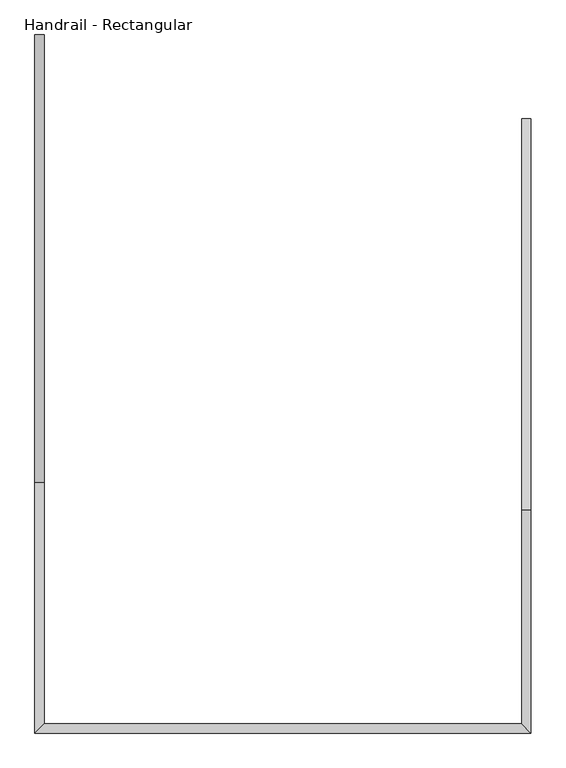
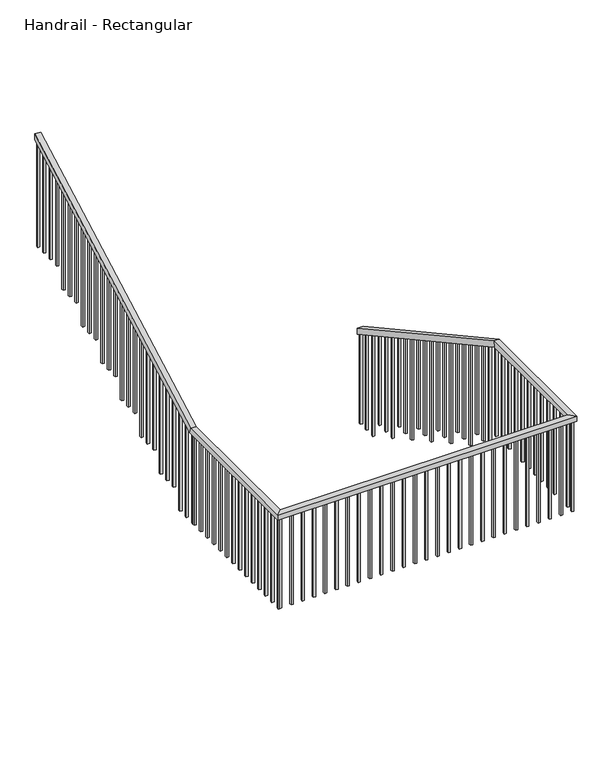
"""IFC4 building model written with IfcOpenShell, lengths in millimetres: railing geometry, Handrail - Rectangular."""

from ifc_helpers import new_model, si_unit, frame, origin, place, context, project, spatial, polyline, outline, extrude, faceted_brep, source, transform, mapped, element, save


def handrail_rectangular_cd72d91a(model_context):
    return source(origin(), model_context, "Body", "SolidModel", [
        faceted_brep([(-73285.35, 12185.65, 17490.1411765), (-73285.35, 12185.65, 17432.1885835), (-73336.15, 12185.65, 17432.1885835), (-73336.15, 12185.65, 17490.1411765), (-73285.35, 10052.05, 18661.5294118), (-73285.35, 10039.0220627, 18610.7294118), (-73336.15, 10039.0220627, 18610.7294118), (-73336.15, 10052.05, 18661.5294118), (-73285.35, 8839.2, 18661.5294118), (-73285.35, 8839.2, 18610.7294118), (-73336.15, 8890.0, 18610.7294118), (-73336.15, 8890.0, 18661.5294118), (-75990.45, 8839.2, 18661.5294118), (-75990.45, 8839.2, 18610.7294118), (-75939.65, 8890.0, 18610.7294118), (-75939.65, 8890.0, 18661.5294118), (-75990.45, 10204.45, 18661.5294118), (-75990.45, 10217.4779373, 18610.7294118), (-75939.65, 10217.4779373, 18610.7294118), (-75939.65, 10204.45, 18661.5294118), (-75990.45, 12642.85, 20000.2588235), (-75939.65, 12642.85, 20000.2588235), (-75939.65, 12642.85, 19942.3062305), (-75990.45, 12642.85, 19942.3062305)], [[[0, 1, 2, 3]], [[1, 0, 4, 5]], [[2, 1, 5, 6]], [[3, 2, 6, 7]], [[0, 3, 7, 4]], [[5, 4, 8, 9]], [[6, 5, 9, 10]], [[7, 6, 10, 11]], [[4, 7, 11, 8]], [[9, 8, 12, 13]], [[10, 9, 13, 14]], [[11, 10, 14, 15]], [[8, 11, 15, 12]], [[13, 12, 16, 17]], [[14, 13, 17, 18]], [[15, 14, 18, 19]], [[12, 15, 19, 16]], [[20, 21, 22, 23]], [[17, 16, 20, 23]], [[18, 17, 23, 22]], [[19, 18, 22, 21]], [[16, 19, 21, 20]]]),
        extrude(outline(polyline([(12550.775, 19891.7552501), (12550.775, 18918.5176471), (12531.725, 18918.5176471), (12531.725, 19881.2964266), (12550.775, 19891.7552501)])), frame((-75974.575, 0.0, 0.0), z_axis=(1.0, 0.0, 0.0), x_axis=(0.0, 1.0, 0.0)), (0.0, 0.0, 1.0), 19.05),
        extrude(outline(polyline([(12449.175, 19835.974858), (12449.175, 18918.5176471), (12430.125, 18918.5176471), (12430.125, 19825.5160344), (12449.175, 19835.974858)])), frame((-75974.575, 0.0, 0.0), z_axis=(1.0, 0.0, 0.0), x_axis=(0.0, 1.0, 0.0)), (0.0, 0.0, 1.0), 19.05),
        extrude(outline(polyline([(12347.575, 19780.1944658), (12347.575, 18918.5176471), (12328.525, 18918.5176471), (12328.525, 19769.7356423), (12347.575, 19780.1944658)])), frame((-75974.575, 0.0, 0.0), z_axis=(1.0, 0.0, 0.0), x_axis=(0.0, 1.0, 0.0)), (0.0, 0.0, 1.0), 19.05),
        extrude(outline(polyline([(12245.975, 19724.4140737), (12245.975, 18751.1764706), (12226.925, 18751.1764706), (12226.925, 19713.9552501), (12245.975, 19724.4140737)])), frame((-75974.575, 0.0, 0.0), z_axis=(1.0, 0.0, 0.0), x_axis=(0.0, 1.0, 0.0)), (0.0, 0.0, 1.0), 19.05),
        extrude(outline(polyline([(12144.375, 19668.6336815), (12144.375, 18751.1764706), (12125.325, 18751.1764706), (12125.325, 19658.174858), (12144.375, 19668.6336815)])), frame((-75974.575, 0.0, 0.0), z_axis=(1.0, 0.0, 0.0), x_axis=(0.0, 1.0, 0.0)), (0.0, 0.0, 1.0), 19.05),
        extrude(outline(polyline([(12042.775, 19612.8532893), (12042.775, 18751.1764706), (12023.725, 18751.1764706), (12023.725, 19602.3944658), (12042.775, 19612.8532893)])), frame((-75974.575, 0.0, 0.0), z_axis=(1.0, 0.0, 0.0), x_axis=(0.0, 1.0, 0.0)), (0.0, 0.0, 1.0), 19.05),
        extrude(outline(polyline([(11941.175, 19557.0728972), (11941.175, 18583.8352941), (11922.125, 18583.8352941), (11922.125, 19546.6140737), (11941.175, 19557.0728972)])), frame((-75974.575, 0.0, 0.0), z_axis=(1.0, 0.0, 0.0), x_axis=(0.0, 1.0, 0.0)), (0.0, 0.0, 1.0), 19.05),
        extrude(outline(polyline([(11839.575, 19501.292505), (11839.575, 18583.8352941), (11820.525, 18583.8352941), (11820.525, 19490.8336815), (11839.575, 19501.292505)])), frame((-75974.575, 0.0, 0.0), z_axis=(1.0, 0.0, 0.0), x_axis=(0.0, 1.0, 0.0)), (0.0, 0.0, 1.0), 19.05),
        extrude(outline(polyline([(11737.975, 19445.5121129), (11737.975, 18583.8352941), (11718.925, 18583.8352941), (11718.925, 19435.0532893), (11737.975, 19445.5121129)])), frame((-75974.575, 0.0, 0.0), z_axis=(1.0, 0.0, 0.0), x_axis=(0.0, 1.0, 0.0)), (0.0, 0.0, 1.0), 19.05),
        extrude(outline(polyline([(11636.375, 19389.7317207), (11636.375, 18416.4941176), (11617.325, 18416.4941176), (11617.325, 19379.2728972), (11636.375, 19389.7317207)])), frame((-75974.575, 0.0, 0.0), z_axis=(1.0, 0.0, 0.0), x_axis=(0.0, 1.0, 0.0)), (0.0, 0.0, 1.0), 19.05),
        extrude(outline(polyline([(11534.775, 19333.9513286), (11534.775, 18416.4941176), (11515.725, 18416.4941176), (11515.725, 19323.492505), (11534.775, 19333.9513286)])), frame((-75974.575, 0.0, 0.0), z_axis=(1.0, 0.0, 0.0), x_axis=(0.0, 1.0, 0.0)), (0.0, 0.0, 1.0), 19.05),
        extrude(outline(polyline([(11433.175, 19278.1709364), (11433.175, 18416.4941176), (11414.125, 18416.4941176), (11414.125, 19267.7121129), (11433.175, 19278.1709364)])), frame((-75974.575, 0.0, 0.0), z_axis=(1.0, 0.0, 0.0), x_axis=(0.0, 1.0, 0.0)), (0.0, 0.0, 1.0), 19.05),
        extrude(outline(polyline([(11331.575, 19222.3905442), (11331.575, 18249.1529412), (11312.525, 18249.1529412), (11312.525, 19211.9317207), (11331.575, 19222.3905442)])), frame((-75974.575, 0.0, 0.0), z_axis=(1.0, 0.0, 0.0), x_axis=(0.0, 1.0, 0.0)), (0.0, 0.0, 1.0), 19.05),
        extrude(outline(polyline([(11229.975, 19166.6101521), (11229.975, 18249.1529412), (11210.925, 18249.1529412), (11210.925, 19156.1513286), (11229.975, 19166.6101521)])), frame((-75974.575, 0.0, 0.0), z_axis=(1.0, 0.0, 0.0), x_axis=(0.0, 1.0, 0.0)), (0.0, 0.0, 1.0), 19.05),
        extrude(outline(polyline([(11128.375, 19110.8297599), (11128.375, 18249.1529412), (11109.325, 18249.1529412), (11109.325, 19100.3709364), (11128.375, 19110.8297599)])), frame((-75974.575, 0.0, 0.0), z_axis=(1.0, 0.0, 0.0), x_axis=(0.0, 1.0, 0.0)), (0.0, 0.0, 1.0), 19.05),
        extrude(outline(polyline([(11026.775, 19055.0493678), (11026.775, 18081.8117647), (11007.725, 18081.8117647), (11007.725, 19044.5905442), (11026.775, 19055.0493678)])), frame((-75974.575, 0.0, 0.0), z_axis=(1.0, 0.0, 0.0), x_axis=(0.0, 1.0, 0.0)), (0.0, 0.0, 1.0), 19.05),
        extrude(outline(polyline([(10925.175, 18999.2689756), (10925.175, 18081.8117647), (10906.125, 18081.8117647), (10906.125, 18988.8101521), (10925.175, 18999.2689756)])), frame((-75974.575, 0.0, 0.0), z_axis=(1.0, 0.0, 0.0), x_axis=(0.0, 1.0, 0.0)), (0.0, 0.0, 1.0), 19.05),
        extrude(outline(polyline([(10823.575, 18943.4885835), (10823.575, 18081.8117647), (10804.525, 18081.8117647), (10804.525, 18933.0297599), (10823.575, 18943.4885835)])), frame((-75974.575, 0.0, 0.0), z_axis=(1.0, 0.0, 0.0), x_axis=(0.0, 1.0, 0.0)), (0.0, 0.0, 1.0), 19.05),
        extrude(outline(polyline([(10721.975, 18887.7081913), (10721.975, 17914.4705882), (10702.925, 17914.4705882), (10702.925, 18877.2493678), (10721.975, 18887.7081913)])), frame((-75974.575, 0.0, 0.0), z_axis=(1.0, 0.0, 0.0), x_axis=(0.0, 1.0, 0.0)), (0.0, 0.0, 1.0), 19.05),
        extrude(outline(polyline([(10620.375, 18831.9277991), (10620.375, 17914.4705882), (10601.325, 17914.4705882), (10601.325, 18821.4689756), (10620.375, 18831.9277991)])), frame((-75974.575, 0.0, 0.0), z_axis=(1.0, 0.0, 0.0), x_axis=(0.0, 1.0, 0.0)), (0.0, 0.0, 1.0), 19.05),
        extrude(outline(polyline([(10518.775, 18776.147407), (10518.775, 17914.4705882), (10499.725, 17914.4705882), (10499.725, 18765.6885835), (10518.775, 18776.147407)])), frame((-75974.575, 0.0, 0.0), z_axis=(1.0, 0.0, 0.0), x_axis=(0.0, 1.0, 0.0)), (0.0, 0.0, 1.0), 19.05),
        extrude(outline(polyline([(10417.175, 18720.3670148), (10417.175, 17747.1294118), (10398.125, 17747.1294118), (10398.125, 18709.9081913), (10417.175, 18720.3670148)])), frame((-75974.575, 0.0, 0.0), z_axis=(1.0, 0.0, 0.0), x_axis=(0.0, 1.0, 0.0)), (0.0, 0.0, 1.0), 19.05),
        extrude(outline(polyline([(10315.575, 18664.5866227), (10315.575, 17747.1294118), (10296.525, 17747.1294118), (10296.525, 18654.1277991), (10315.575, 18664.5866227)])), frame((-75974.575, 0.0, 0.0), z_axis=(1.0, 0.0, 0.0), x_axis=(0.0, 1.0, 0.0)), (0.0, 0.0, 1.0), 19.05),
        extrude(outline(polyline([(-75974.575, 10175.875), (-75974.575, 10194.925), (-75955.525, 10194.925), (-75955.525, 10175.875), (-75974.575, 10175.875)])), frame((0.0, 0.0, 17747.1294118), z_axis=(0.0, 0.0, 1.0), x_axis=(1.0, 0.0, 0.0)), (0.0, 0.0, 1.0), 863.6),
        extrude(outline(polyline([(-75974.575, 10074.275), (-75974.575, 10093.325), (-75955.525, 10093.325), (-75955.525, 10074.275), (-75974.575, 10074.275)])), frame((0.0, 0.0, 17747.1294118), z_axis=(0.0, 0.0, 1.0), x_axis=(1.0, 0.0, 0.0)), (0.0, 0.0, 1.0), 863.6),
        extrude(outline(polyline([(-75974.575, 9972.675), (-75974.575, 9991.725), (-75955.525, 9991.725), (-75955.525, 9972.675), (-75974.575, 9972.675)])), frame((0.0, 0.0, 17747.1294118), z_axis=(0.0, 0.0, 1.0), x_axis=(1.0, 0.0, 0.0)), (0.0, 0.0, 1.0), 863.6),
        extrude(outline(polyline([(-75974.575, 9871.075), (-75974.575, 9890.125), (-75955.525, 9890.125), (-75955.525, 9871.075), (-75974.575, 9871.075)])), frame((0.0, 0.0, 17747.1294118), z_axis=(0.0, 0.0, 1.0), x_axis=(1.0, 0.0, 0.0)), (0.0, 0.0, 1.0), 863.6),
        extrude(outline(polyline([(-75974.575, 9769.475), (-75974.575, 9788.525), (-75955.525, 9788.525), (-75955.525, 9769.475), (-75974.575, 9769.475)])), frame((0.0, 0.0, 17747.1294118), z_axis=(0.0, 0.0, 1.0), x_axis=(1.0, 0.0, 0.0)), (0.0, 0.0, 1.0), 863.6),
        extrude(outline(polyline([(-75974.575, 9667.875), (-75974.575, 9686.925), (-75955.525, 9686.925), (-75955.525, 9667.875), (-75974.575, 9667.875)])), frame((0.0, 0.0, 17747.1294118), z_axis=(0.0, 0.0, 1.0), x_axis=(1.0, 0.0, 0.0)), (0.0, 0.0, 1.0), 863.6),
        extrude(outline(polyline([(-75974.575, 9566.275), (-75974.575, 9585.325), (-75955.525, 9585.325), (-75955.525, 9566.275), (-75974.575, 9566.275)])), frame((0.0, 0.0, 17747.1294118), z_axis=(0.0, 0.0, 1.0), x_axis=(1.0, 0.0, 0.0)), (0.0, 0.0, 1.0), 863.6),
        extrude(outline(polyline([(-75974.575, 9464.675), (-75974.575, 9483.725), (-75955.525, 9483.725), (-75955.525, 9464.675), (-75974.575, 9464.675)])), frame((0.0, 0.0, 17747.1294118), z_axis=(0.0, 0.0, 1.0), x_axis=(1.0, 0.0, 0.0)), (0.0, 0.0, 1.0), 863.6),
        extrude(outline(polyline([(-75974.575, 9363.075), (-75974.575, 9382.125), (-75955.525, 9382.125), (-75955.525, 9363.075), (-75974.575, 9363.075)])), frame((0.0, 0.0, 17747.1294118), z_axis=(0.0, 0.0, 1.0), x_axis=(1.0, 0.0, 0.0)), (0.0, 0.0, 1.0), 863.6),
        extrude(outline(polyline([(-75974.575, 9261.475), (-75974.575, 9280.525), (-75955.525, 9280.525), (-75955.525, 9261.475), (-75974.575, 9261.475)])), frame((0.0, 0.0, 17747.1294118), z_axis=(0.0, 0.0, 1.0), x_axis=(1.0, 0.0, 0.0)), (0.0, 0.0, 1.0), 863.6),
        extrude(outline(polyline([(-75974.575, 9159.875), (-75974.575, 9178.925), (-75955.525, 9178.925), (-75955.525, 9159.875), (-75974.575, 9159.875)])), frame((0.0, 0.0, 17747.1294118), z_axis=(0.0, 0.0, 1.0), x_axis=(1.0, 0.0, 0.0)), (0.0, 0.0, 1.0), 863.6),
        extrude(outline(polyline([(-75974.575, 9058.275), (-75974.575, 9077.325), (-75955.525, 9077.325), (-75955.525, 9058.275), (-75974.575, 9058.275)])), frame((0.0, 0.0, 17747.1294118), z_axis=(0.0, 0.0, 1.0), x_axis=(1.0, 0.0, 0.0)), (0.0, 0.0, 1.0), 863.6),
        extrude(outline(polyline([(-75974.575, 8956.675), (-75974.575, 8975.725), (-75955.525, 8975.725), (-75955.525, 8956.675), (-75974.575, 8956.675)])), frame((0.0, 0.0, 17747.1294118), z_axis=(0.0, 0.0, 1.0), x_axis=(1.0, 0.0, 0.0)), (0.0, 0.0, 1.0), 863.6),
        extrude(outline(polyline([(-75942.825, 8855.075), (-75961.875, 8855.075), (-75961.875, 8874.125), (-75942.825, 8874.125), (-75942.825, 8855.075)])), frame((0.0, 0.0, 17747.1294118), z_axis=(0.0, 0.0, 1.0), x_axis=(1.0, 0.0, 0.0)), (0.0, 0.0, 1.0), 863.6),
        extrude(outline(polyline([(-75841.225, 8855.075), (-75860.275, 8855.075), (-75860.275, 8874.125), (-75841.225, 8874.125), (-75841.225, 8855.075)])), frame((0.0, 0.0, 17747.1294118), z_axis=(0.0, 0.0, 1.0), x_axis=(1.0, 0.0, 0.0)), (0.0, 0.0, 1.0), 863.6),
        extrude(outline(polyline([(-75739.625, 8855.075), (-75758.675, 8855.075), (-75758.675, 8874.125), (-75739.625, 8874.125), (-75739.625, 8855.075)])), frame((0.0, 0.0, 17747.1294118), z_axis=(0.0, 0.0, 1.0), x_axis=(1.0, 0.0, 0.0)), (0.0, 0.0, 1.0), 863.6),
        extrude(outline(polyline([(-75638.025, 8855.075), (-75657.075, 8855.075), (-75657.075, 8874.125), (-75638.025, 8874.125), (-75638.025, 8855.075)])), frame((0.0, 0.0, 17747.1294118), z_axis=(0.0, 0.0, 1.0), x_axis=(1.0, 0.0, 0.0)), (0.0, 0.0, 1.0), 863.6),
        extrude(outline(polyline([(-75536.425, 8855.075), (-75555.475, 8855.075), (-75555.475, 8874.125), (-75536.425, 8874.125), (-75536.425, 8855.075)])), frame((0.0, 0.0, 17747.1294118), z_axis=(0.0, 0.0, 1.0), x_axis=(1.0, 0.0, 0.0)), (0.0, 0.0, 1.0), 863.6),
        extrude(outline(polyline([(-75434.825, 8855.075), (-75453.875, 8855.075), (-75453.875, 8874.125), (-75434.825, 8874.125), (-75434.825, 8855.075)])), frame((0.0, 0.0, 17747.1294118), z_axis=(0.0, 0.0, 1.0), x_axis=(1.0, 0.0, 0.0)), (0.0, 0.0, 1.0), 863.6),
        extrude(outline(polyline([(-75333.225, 8855.075), (-75352.275, 8855.075), (-75352.275, 8874.125), (-75333.225, 8874.125), (-75333.225, 8855.075)])), frame((0.0, 0.0, 17747.1294118), z_axis=(0.0, 0.0, 1.0), x_axis=(1.0, 0.0, 0.0)), (0.0, 0.0, 1.0), 863.6),
        extrude(outline(polyline([(-75231.625, 8855.075), (-75250.675, 8855.075), (-75250.675, 8874.125), (-75231.625, 8874.125), (-75231.625, 8855.075)])), frame((0.0, 0.0, 17747.1294118), z_axis=(0.0, 0.0, 1.0), x_axis=(1.0, 0.0, 0.0)), (0.0, 0.0, 1.0), 863.6),
        extrude(outline(polyline([(-75130.025, 8855.075), (-75149.075, 8855.075), (-75149.075, 8874.125), (-75130.025, 8874.125), (-75130.025, 8855.075)])), frame((0.0, 0.0, 17747.1294118), z_axis=(0.0, 0.0, 1.0), x_axis=(1.0, 0.0, 0.0)), (0.0, 0.0, 1.0), 863.6),
        extrude(outline(polyline([(-75028.425, 8855.075), (-75047.475, 8855.075), (-75047.475, 8874.125), (-75028.425, 8874.125), (-75028.425, 8855.075)])), frame((0.0, 0.0, 17747.1294118), z_axis=(0.0, 0.0, 1.0), x_axis=(1.0, 0.0, 0.0)), (0.0, 0.0, 1.0), 863.6),
        extrude(outline(polyline([(-74926.825, 8855.075), (-74945.875, 8855.075), (-74945.875, 8874.125), (-74926.825, 8874.125), (-74926.825, 8855.075)])), frame((0.0, 0.0, 17747.1294118), z_axis=(0.0, 0.0, 1.0), x_axis=(1.0, 0.0, 0.0)), (0.0, 0.0, 1.0), 863.6),
        extrude(outline(polyline([(-74825.225, 8855.075), (-74844.275, 8855.075), (-74844.275, 8874.125), (-74825.225, 8874.125), (-74825.225, 8855.075)])), frame((0.0, 0.0, 17747.1294118), z_axis=(0.0, 0.0, 1.0), x_axis=(1.0, 0.0, 0.0)), (0.0, 0.0, 1.0), 863.6),
        extrude(outline(polyline([(-74723.625, 8855.075), (-74742.675, 8855.075), (-74742.675, 8874.125), (-74723.625, 8874.125), (-74723.625, 8855.075)])), frame((0.0, 0.0, 17747.1294118), z_axis=(0.0, 0.0, 1.0), x_axis=(1.0, 0.0, 0.0)), (0.0, 0.0, 1.0), 863.6),
        extrude(outline(polyline([(-74622.025, 8855.075), (-74641.075, 8855.075), (-74641.075, 8874.125), (-74622.025, 8874.125), (-74622.025, 8855.075)])), frame((0.0, 0.0, 17747.1294118), z_axis=(0.0, 0.0, 1.0), x_axis=(1.0, 0.0, 0.0)), (0.0, 0.0, 1.0), 863.6),
        extrude(outline(polyline([(-74520.425, 8855.075), (-74539.475, 8855.075), (-74539.475, 8874.125), (-74520.425, 8874.125), (-74520.425, 8855.075)])), frame((0.0, 0.0, 17747.1294118), z_axis=(0.0, 0.0, 1.0), x_axis=(1.0, 0.0, 0.0)), (0.0, 0.0, 1.0), 863.6),
        extrude(outline(polyline([(-74418.825, 8855.075), (-74437.875, 8855.075), (-74437.875, 8874.125), (-74418.825, 8874.125), (-74418.825, 8855.075)])), frame((0.0, 0.0, 17747.1294118), z_axis=(0.0, 0.0, 1.0), x_axis=(1.0, 0.0, 0.0)), (0.0, 0.0, 1.0), 863.6),
        extrude(outline(polyline([(-74317.225, 8855.075), (-74336.275, 8855.075), (-74336.275, 8874.125), (-74317.225, 8874.125), (-74317.225, 8855.075)])), frame((0.0, 0.0, 17747.1294118), z_axis=(0.0, 0.0, 1.0), x_axis=(1.0, 0.0, 0.0)), (0.0, 0.0, 1.0), 863.6),
        extrude(outline(polyline([(-74215.625, 8855.075), (-74234.675, 8855.075), (-74234.675, 8874.125), (-74215.625, 8874.125), (-74215.625, 8855.075)])), frame((0.0, 0.0, 17747.1294118), z_axis=(0.0, 0.0, 1.0), x_axis=(1.0, 0.0, 0.0)), (0.0, 0.0, 1.0), 863.6),
        extrude(outline(polyline([(-74114.025, 8855.075), (-74133.075, 8855.075), (-74133.075, 8874.125), (-74114.025, 8874.125), (-74114.025, 8855.075)])), frame((0.0, 0.0, 17747.1294118), z_axis=(0.0, 0.0, 1.0), x_axis=(1.0, 0.0, 0.0)), (0.0, 0.0, 1.0), 863.6),
        extrude(outline(polyline([(-74012.425, 8855.075), (-74031.475, 8855.075), (-74031.475, 8874.125), (-74012.425, 8874.125), (-74012.425, 8855.075)])), frame((0.0, 0.0, 17747.1294118), z_axis=(0.0, 0.0, 1.0), x_axis=(1.0, 0.0, 0.0)), (0.0, 0.0, 1.0), 863.6),
        extrude(outline(polyline([(-73910.825, 8855.075), (-73929.875, 8855.075), (-73929.875, 8874.125), (-73910.825, 8874.125), (-73910.825, 8855.075)])), frame((0.0, 0.0, 17747.1294118), z_axis=(0.0, 0.0, 1.0), x_axis=(1.0, 0.0, 0.0)), (0.0, 0.0, 1.0), 863.6),
        extrude(outline(polyline([(-73809.225, 8855.075), (-73828.275, 8855.075), (-73828.275, 8874.125), (-73809.225, 8874.125), (-73809.225, 8855.075)])), frame((0.0, 0.0, 17747.1294118), z_axis=(0.0, 0.0, 1.0), x_axis=(1.0, 0.0, 0.0)), (0.0, 0.0, 1.0), 863.6),
        extrude(outline(polyline([(-73707.625, 8855.075), (-73726.675, 8855.075), (-73726.675, 8874.125), (-73707.625, 8874.125), (-73707.625, 8855.075)])), frame((0.0, 0.0, 17747.1294118), z_axis=(0.0, 0.0, 1.0), x_axis=(1.0, 0.0, 0.0)), (0.0, 0.0, 1.0), 863.6),
        extrude(outline(polyline([(-73606.025, 8855.075), (-73625.075, 8855.075), (-73625.075, 8874.125), (-73606.025, 8874.125), (-73606.025, 8855.075)])), frame((0.0, 0.0, 17747.1294118), z_axis=(0.0, 0.0, 1.0), x_axis=(1.0, 0.0, 0.0)), (0.0, 0.0, 1.0), 863.6),
        extrude(outline(polyline([(-73504.425, 8855.075), (-73523.475, 8855.075), (-73523.475, 8874.125), (-73504.425, 8874.125), (-73504.425, 8855.075)])), frame((0.0, 0.0, 17747.1294118), z_axis=(0.0, 0.0, 1.0), x_axis=(1.0, 0.0, 0.0)), (0.0, 0.0, 1.0), 863.6),
        extrude(outline(polyline([(-73402.825, 8855.075), (-73421.875, 8855.075), (-73421.875, 8874.125), (-73402.825, 8874.125), (-73402.825, 8855.075)])), frame((0.0, 0.0, 17747.1294118), z_axis=(0.0, 0.0, 1.0), x_axis=(1.0, 0.0, 0.0)), (0.0, 0.0, 1.0), 863.6),
        extrude(outline(polyline([(-73301.225, 8943.975), (-73301.225, 8924.925), (-73320.275, 8924.925), (-73320.275, 8943.975), (-73301.225, 8943.975)])), frame((0.0, 0.0, 17747.1294118), z_axis=(0.0, 0.0, 1.0), x_axis=(1.0, 0.0, 0.0)), (0.0, 0.0, 1.0), 863.6),
        extrude(outline(polyline([(-73301.225, 9045.575), (-73301.225, 9026.525), (-73320.275, 9026.525), (-73320.275, 9045.575), (-73301.225, 9045.575)])), frame((0.0, 0.0, 17747.1294118), z_axis=(0.0, 0.0, 1.0), x_axis=(1.0, 0.0, 0.0)), (0.0, 0.0, 1.0), 863.6),
        extrude(outline(polyline([(-73301.225, 9147.175), (-73301.225, 9128.125), (-73320.275, 9128.125), (-73320.275, 9147.175), (-73301.225, 9147.175)])), frame((0.0, 0.0, 17747.1294118), z_axis=(0.0, 0.0, 1.0), x_axis=(1.0, 0.0, 0.0)), (0.0, 0.0, 1.0), 863.6),
        extrude(outline(polyline([(-73301.225, 9248.775), (-73301.225, 9229.725), (-73320.275, 9229.725), (-73320.275, 9248.775), (-73301.225, 9248.775)])), frame((0.0, 0.0, 17747.1294118), z_axis=(0.0, 0.0, 1.0), x_axis=(1.0, 0.0, 0.0)), (0.0, 0.0, 1.0), 863.6),
        extrude(outline(polyline([(-73301.225, 9350.375), (-73301.225, 9331.325), (-73320.275, 9331.325), (-73320.275, 9350.375), (-73301.225, 9350.375)])), frame((0.0, 0.0, 17747.1294118), z_axis=(0.0, 0.0, 1.0), x_axis=(1.0, 0.0, 0.0)), (0.0, 0.0, 1.0), 863.6),
        extrude(outline(polyline([(-73301.225, 9451.975), (-73301.225, 9432.925), (-73320.275, 9432.925), (-73320.275, 9451.975), (-73301.225, 9451.975)])), frame((0.0, 0.0, 17747.1294118), z_axis=(0.0, 0.0, 1.0), x_axis=(1.0, 0.0, 0.0)), (0.0, 0.0, 1.0), 863.6),
        extrude(outline(polyline([(-73301.225, 9553.575), (-73301.225, 9534.525), (-73320.275, 9534.525), (-73320.275, 9553.575), (-73301.225, 9553.575)])), frame((0.0, 0.0, 17747.1294118), z_axis=(0.0, 0.0, 1.0), x_axis=(1.0, 0.0, 0.0)), (0.0, 0.0, 1.0), 863.6),
        extrude(outline(polyline([(-73301.225, 9655.175), (-73301.225, 9636.125), (-73320.275, 9636.125), (-73320.275, 9655.175), (-73301.225, 9655.175)])), frame((0.0, 0.0, 17747.1294118), z_axis=(0.0, 0.0, 1.0), x_axis=(1.0, 0.0, 0.0)), (0.0, 0.0, 1.0), 863.6),
        extrude(outline(polyline([(-73301.225, 9756.775), (-73301.225, 9737.725), (-73320.275, 9737.725), (-73320.275, 9756.775), (-73301.225, 9756.775)])), frame((0.0, 0.0, 17747.1294118), z_axis=(0.0, 0.0, 1.0), x_axis=(1.0, 0.0, 0.0)), (0.0, 0.0, 1.0), 863.6),
        extrude(outline(polyline([(-73301.225, 9858.375), (-73301.225, 9839.325), (-73320.275, 9839.325), (-73320.275, 9858.375), (-73301.225, 9858.375)])), frame((0.0, 0.0, 17747.1294118), z_axis=(0.0, 0.0, 1.0), x_axis=(1.0, 0.0, 0.0)), (0.0, 0.0, 1.0), 863.6),
        extrude(outline(polyline([(-73301.225, 9959.975), (-73301.225, 9940.925), (-73320.275, 9940.925), (-73320.275, 9959.975), (-73301.225, 9959.975)])), frame((0.0, 0.0, 17747.1294118), z_axis=(0.0, 0.0, 1.0), x_axis=(1.0, 0.0, 0.0)), (0.0, 0.0, 1.0), 863.6),
        extrude(outline(polyline([(10163.175, 18542.5670148), (10163.175, 17579.7882353), (10144.125, 17579.7882353), (10144.125, 18553.0258384), (10163.175, 18542.5670148)])), frame((-73320.275, 0.0, 0.0), z_axis=(1.0, 0.0, 0.0), x_axis=(0.0, 1.0, 0.0)), (0.0, 0.0, 1.0), 19.05),
        extrude(outline(polyline([(10264.775, 18486.7866227), (10264.775, 17579.7882353), (10245.725, 17579.7882353), (10245.725, 18497.2454462), (10264.775, 18486.7866227)])), frame((-73320.275, 0.0, 0.0), z_axis=(1.0, 0.0, 0.0), x_axis=(0.0, 1.0, 0.0)), (0.0, 0.0, 1.0), 19.05),
        extrude(outline(polyline([(10366.375, 18431.0062305), (10366.375, 17579.7882353), (10347.325, 17579.7882353), (10347.325, 18441.465054), (10366.375, 18431.0062305)])), frame((-73320.275, 0.0, 0.0), z_axis=(1.0, 0.0, 0.0), x_axis=(0.0, 1.0, 0.0)), (0.0, 0.0, 1.0), 19.05),
        extrude(outline(polyline([(10467.975, 18375.2258384), (10467.975, 17412.4470588), (10448.925, 17412.4470588), (10448.925, 18385.6846619), (10467.975, 18375.2258384)])), frame((-73320.275, 0.0, 0.0), z_axis=(1.0, 0.0, 0.0), x_axis=(0.0, 1.0, 0.0)), (0.0, 0.0, 1.0), 19.05),
        extrude(outline(polyline([(10569.575, 18319.4454462), (10569.575, 17412.4470588), (10550.525, 17412.4470588), (10550.525, 18329.9042697), (10569.575, 18319.4454462)])), frame((-73320.275, 0.0, 0.0), z_axis=(1.0, 0.0, 0.0), x_axis=(0.0, 1.0, 0.0)), (0.0, 0.0, 1.0), 19.05),
        extrude(outline(polyline([(10671.175, 18263.665054), (10671.175, 17412.4470588), (10652.125, 17412.4470588), (10652.125, 18274.1238776), (10671.175, 18263.665054)])), frame((-73320.275, 0.0, 0.0), z_axis=(1.0, 0.0, 0.0), x_axis=(0.0, 1.0, 0.0)), (0.0, 0.0, 1.0), 19.05),
        extrude(outline(polyline([(10772.775, 18207.8846619), (10772.775, 17245.1058824), (10753.725, 17245.1058824), (10753.725, 18218.3434854), (10772.775, 18207.8846619)])), frame((-73320.275, 0.0, 0.0), z_axis=(1.0, 0.0, 0.0), x_axis=(0.0, 1.0, 0.0)), (0.0, 0.0, 1.0), 19.05),
        extrude(outline(polyline([(10874.375, 18152.1042697), (10874.375, 17245.1058824), (10855.325, 17245.1058824), (10855.325, 18162.5630933), (10874.375, 18152.1042697)])), frame((-73320.275, 0.0, 0.0), z_axis=(1.0, 0.0, 0.0), x_axis=(0.0, 1.0, 0.0)), (0.0, 0.0, 1.0), 19.05),
        extrude(outline(polyline([(10975.975, 18096.3238776), (10975.975, 17245.1058824), (10956.925, 17245.1058824), (10956.925, 18106.7827011), (10975.975, 18096.3238776)])), frame((-73320.275, 0.0, 0.0), z_axis=(1.0, 0.0, 0.0), x_axis=(0.0, 1.0, 0.0)), (0.0, 0.0, 1.0), 19.05),
        extrude(outline(polyline([(11077.575, 18040.5434854), (11077.575, 17077.7647059), (11058.525, 17077.7647059), (11058.525, 18051.0023089), (11077.575, 18040.5434854)])), frame((-73320.275, 0.0, 0.0), z_axis=(1.0, 0.0, 0.0), x_axis=(0.0, 1.0, 0.0)), (0.0, 0.0, 1.0), 19.05),
        extrude(outline(polyline([(11179.175, 17984.7630933), (11179.175, 17077.7647059), (11160.125, 17077.7647059), (11160.125, 17995.2219168), (11179.175, 17984.7630933)])), frame((-73320.275, 0.0, 0.0), z_axis=(1.0, 0.0, 0.0), x_axis=(0.0, 1.0, 0.0)), (0.0, 0.0, 1.0), 19.05),
        extrude(outline(polyline([(11280.775, 17928.9827011), (11280.775, 17077.7647059), (11261.725, 17077.7647059), (11261.725, 17939.4415246), (11280.775, 17928.9827011)])), frame((-73320.275, 0.0, 0.0), z_axis=(1.0, 0.0, 0.0), x_axis=(0.0, 1.0, 0.0)), (0.0, 0.0, 1.0), 19.05),
        extrude(outline(polyline([(11382.375, 17873.2023089), (11382.375, 16910.4235294), (11363.325, 16910.4235294), (11363.325, 17883.6611325), (11382.375, 17873.2023089)])), frame((-73320.275, 0.0, 0.0), z_axis=(1.0, 0.0, 0.0), x_axis=(0.0, 1.0, 0.0)), (0.0, 0.0, 1.0), 19.05),
        extrude(outline(polyline([(11483.975, 17817.4219168), (11483.975, 16910.4235294), (11464.925, 16910.4235294), (11464.925, 17827.8807403), (11483.975, 17817.4219168)])), frame((-73320.275, 0.0, 0.0), z_axis=(1.0, 0.0, 0.0), x_axis=(0.0, 1.0, 0.0)), (0.0, 0.0, 1.0), 19.05),
        extrude(outline(polyline([(11585.575, 17761.6415246), (11585.575, 16910.4235294), (11566.525, 16910.4235294), (11566.525, 17772.1003482), (11585.575, 17761.6415246)])), frame((-73320.275, 0.0, 0.0), z_axis=(1.0, 0.0, 0.0), x_axis=(0.0, 1.0, 0.0)), (0.0, 0.0, 1.0), 19.05),
        extrude(outline(polyline([(11687.175, 17705.8611325), (11687.175, 16743.0823529), (11668.125, 16743.0823529), (11668.125, 17716.319956), (11687.175, 17705.8611325)])), frame((-73320.275, 0.0, 0.0), z_axis=(1.0, 0.0, 0.0), x_axis=(0.0, 1.0, 0.0)), (0.0, 0.0, 1.0), 19.05),
        extrude(outline(polyline([(11788.775, 17650.0807403), (11788.775, 16743.0823529), (11769.725, 16743.0823529), (11769.725, 17660.5395638), (11788.775, 17650.0807403)])), frame((-73320.275, 0.0, 0.0), z_axis=(1.0, 0.0, 0.0), x_axis=(0.0, 1.0, 0.0)), (0.0, 0.0, 1.0), 19.05),
        extrude(outline(polyline([(11890.375, 17594.3003482), (11890.375, 16743.0823529), (11871.325, 16743.0823529), (11871.325, 17604.7591717), (11890.375, 17594.3003482)])), frame((-73320.275, 0.0, 0.0), z_axis=(1.0, 0.0, 0.0), x_axis=(0.0, 1.0, 0.0)), (0.0, 0.0, 1.0), 19.05),
        extrude(outline(polyline([(11991.975, 17538.519956), (11991.975, 16575.7411765), (11972.925, 16575.7411765), (11972.925, 17548.9787795), (11991.975, 17538.519956)])), frame((-73320.275, 0.0, 0.0), z_axis=(1.0, 0.0, 0.0), x_axis=(0.0, 1.0, 0.0)), (0.0, 0.0, 1.0), 19.05),
        extrude(outline(polyline([(12093.575, 17482.7395638), (12093.575, 16575.7411765), (12074.525, 16575.7411765), (12074.525, 17493.1983874), (12093.575, 17482.7395638)])), frame((-73320.275, 0.0, 0.0), z_axis=(1.0, 0.0, 0.0), x_axis=(0.0, 1.0, 0.0)), (0.0, 0.0, 1.0), 19.05),
        extrude(outline(polyline([(-75974.575, 10194.925), (-75974.575, 10213.975), (-75955.525, 10213.975), (-75955.525, 10194.925), (-75974.575, 10194.925)])), frame((0.0, 0.0, 17747.1294118), z_axis=(0.0, 0.0, 1.0), x_axis=(1.0, 0.0, 0.0)), (0.0, 0.0, 1.0), 863.6),
        extrude(outline(polyline([(-75955.525, 8855.075), (-75974.575, 8855.075), (-75974.575, 8874.125), (-75955.525, 8874.125), (-75955.525, 8855.075)])), frame((0.0, 0.0, 17747.1294118), z_axis=(0.0, 0.0, 1.0), x_axis=(1.0, 0.0, 0.0)), (0.0, 0.0, 1.0), 863.6),
        extrude(outline(polyline([(-73301.225, 8874.125), (-73301.225, 8855.075), (-73320.275, 8855.075), (-73320.275, 8874.125), (-73301.225, 8874.125)])), frame((0.0, 0.0, 17747.1294118), z_axis=(0.0, 0.0, 1.0), x_axis=(1.0, 0.0, 0.0)), (0.0, 0.0, 1.0), 863.6),
        extrude(outline(polyline([(10061.575, 18598.347407), (10061.575, 17747.1294118), (10042.525, 17747.1294118), (10042.525, 18608.8062305), (10061.575, 18598.347407)])), frame((-73320.275, 0.0, 0.0), z_axis=(1.0, 0.0, 0.0), x_axis=(0.0, 1.0, 0.0)), (0.0, 0.0, 1.0), 19.05),
        extrude(outline(polyline([(12642.85, 19942.3062305), (12642.85, 18918.5176471), (12623.8, 18918.5176471), (12623.8, 19931.847407), (12642.85, 19942.3062305)])), frame((-75974.575, 0.0, 0.0), z_axis=(1.0, 0.0, 0.0), x_axis=(0.0, 1.0, 0.0)), (0.0, 0.0, 1.0), 19.05),
        extrude(outline(polyline([(12185.65, 17432.1885835), (12185.65, 16575.7411765), (12166.6, 16575.7411765), (12166.6, 17442.647407), (12185.65, 17432.1885835)])), frame((-73320.275, 0.0, 0.0), z_axis=(1.0, 0.0, 0.0), x_axis=(0.0, 1.0, 0.0)), (0.0, 0.0, 1.0), 19.05),
    ])


if __name__ == "__main__":
    model = new_model("IFC4")
    model_context = context("Model", 3, world=origin())
    ifc_project = project(units=[si_unit("LENGTHUNIT", "METRE", prefix="MILLI")], contexts=[model_context])
    site = spatial("IfcSite", under=ifc_project)
    building = spatial("IfcBuilding", under=site)
    placement = place(None, origin())
    handrail_rectangular_shape = handrail_rectangular_cd72d91a(model_context)
    element("IfcRailing", 1, ObjectType="Handrail - Rectangular", at=placement, inside=building, context=model_context, shape_type="MappedRepresentation", body=[
        mapped(handrail_rectangular_shape, transform((0.0, 0.0, 0.0), x_axis=(1.0, 0.0, 0.0), y_axis=(0.0, 1.0, 0.0), z_axis=(0.0, 0.0, 1.0))),
    ])
    save(model, "model.ifc")
